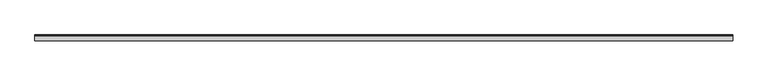
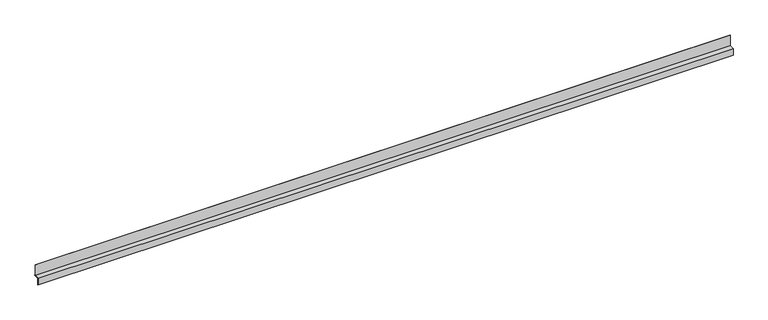
"""IFC4 building model written with IfcOpenShell, lengths in millimetres: proxy geometry, Footer002 : Footer002."""

from ifc_helpers import new_model, si_unit, frame, origin, place, context, project, spatial, polyline, outline, extrude, source, transform, mapped, element, save


def generic_models_0bc8ec64(model_context):
    return source(origin(), model_context, "Body", "SweptSolid", [
        extrude(outline(polyline([(-4248.9225368, 40150.796), (-4250.1925368, 40150.796), (-4250.1925368, 40171.166), (-4235.9042972, 40171.166), (-4235.9042972, 40202.916), (-4234.6342972, 40202.916), (-4234.6342972, 40171.166), (-4233.8244501, 40171.166), (-4233.8244501, 40169.896), (-4248.9225368, 40169.896), (-4248.9225368, 40150.796)])), frame((12383.0178845, 0.0, 0.0), z_axis=(1.0, 0.0, 0.0), x_axis=(0.0, 1.0, 0.0)), (0.0, 0.0, 1.0), 2000.0),
    ])


if __name__ == "__main__":
    model = new_model("IFC4")
    model_context = context("Model", 3, world=origin())
    ifc_project = project(units=[si_unit("LENGTHUNIT", "METRE", prefix="MILLI")], contexts=[model_context])
    site = spatial("IfcSite", under=ifc_project)
    building = spatial("IfcBuilding", under=site)
    placement = place(None, origin())
    generic_models_shape = generic_models_0bc8ec64(model_context)
    element("IfcBuildingElementProxy", 1, Name="Footer002 : Footer002", ObjectType="Footer002 : Footer002", at=placement, inside=building, context=model_context, shape_type="MappedRepresentation", body=[
        mapped(generic_models_shape, transform((0.0, 0.0, 0.0), x_axis=(1.0, 0.0, 0.0), y_axis=(0.0, 1.0, 0.0), z_axis=(0.0, 0.0, 1.0))),
    ])
    save(model, "model.ifc")

# Revit data of these elements
# Type "Footer002 : Footer002"
#   NameOverride = "Footer002"
# Element 1 (IfcBuildingElementProxy, "Footer002 : Footer002")
#   Materials on its faces: "SHADOW Z REVEAL  BEAD"
# Materials
#   "SHADOW Z REVEAL  BEAD": class "Unassigned", colour RGB 251 232 155, transparency 0, Cost = 0
